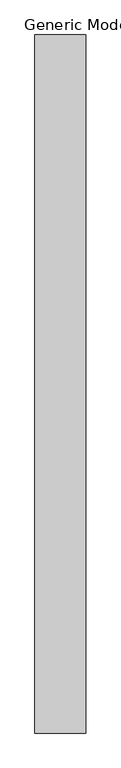
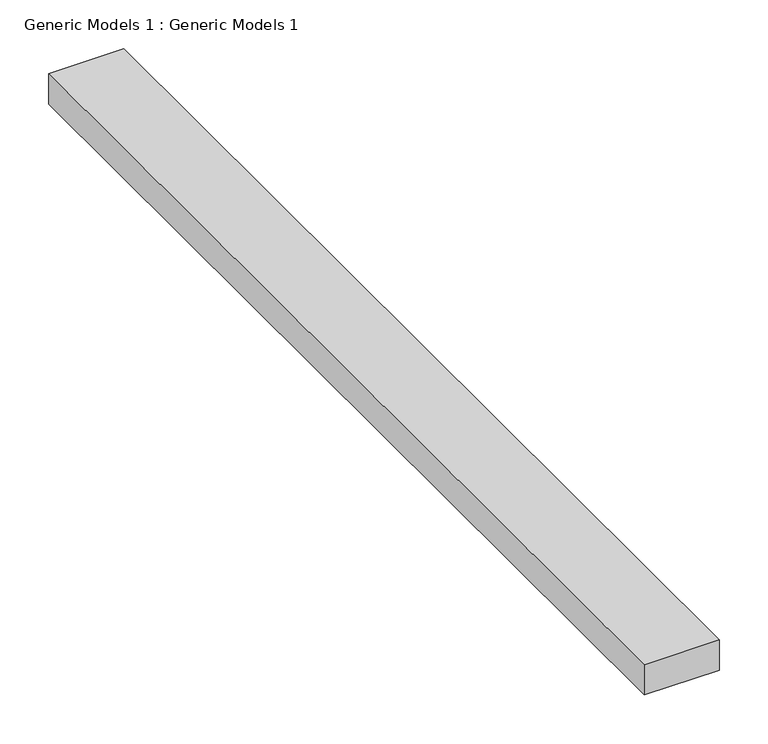
"""IFC4 building model written with IfcOpenShell, lengths in millimetres: proxy geometry, Generic Models 1 : Generic Models 1."""

from ifc_helpers import new_model, si_unit, frame, origin, place, context, project, spatial, polyline, outline, extrude, source, transform, mapped, element, save


def generic_models_1_generic_models_1_05f3df34(model_context):
    return source(origin(), model_context, "Body", "SweptSolid", [
        extrude(outline(polyline([(49784.0, 0.0), (49695.1, 0.0), (49695.1, 1219.2), (49784.0, 1219.2), (49784.0, 0.0)])), frame((0.0, 0.0, 3048.0), z_axis=(0.0, 0.0, 1.0), x_axis=(1.0, 0.0, 0.0)), (0.0, 0.0, 1.0), 38.1),
    ])


if __name__ == "__main__":
    model = new_model("IFC4")
    model_context = context("Model", 3, world=origin())
    ifc_project = project(units=[si_unit("LENGTHUNIT", "METRE", prefix="MILLI")], contexts=[model_context])
    site = spatial("IfcSite", under=ifc_project)
    building = spatial("IfcBuilding", under=site)
    placement = place(None, origin())
    generic_models_1_generic_models_1_shape = generic_models_1_generic_models_1_05f3df34(model_context)
    element("IfcBuildingElementProxy", 1, Name="Generic Models 1 : Generic Models 1", ObjectType="Generic Models 1 : Generic Models 1", at=placement, inside=building, context=model_context, shape_type="MappedRepresentation", body=[
        mapped(generic_models_1_generic_models_1_shape, transform((0.0, 0.0, 0.0), x_axis=(1.0, 0.0, 0.0), y_axis=(0.0, 1.0, 0.0), z_axis=(0.0, 0.0, 1.0))),
    ])
    save(model, "model.ifc")

# Revit data of these elements
# Element 1 (IfcBuildingElementProxy, "Generic Models 1 : Generic Models 1")
#   Materials on its faces: "TREATED 2X WOOD SILL"
# Materials
#   "TREATED 2X WOOD SILL": class "Wood", colour RGB 234 198 147, transparency 0, Description = "Pinus Echinata", Cost = 0
